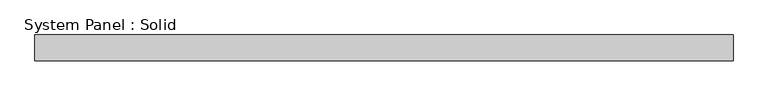
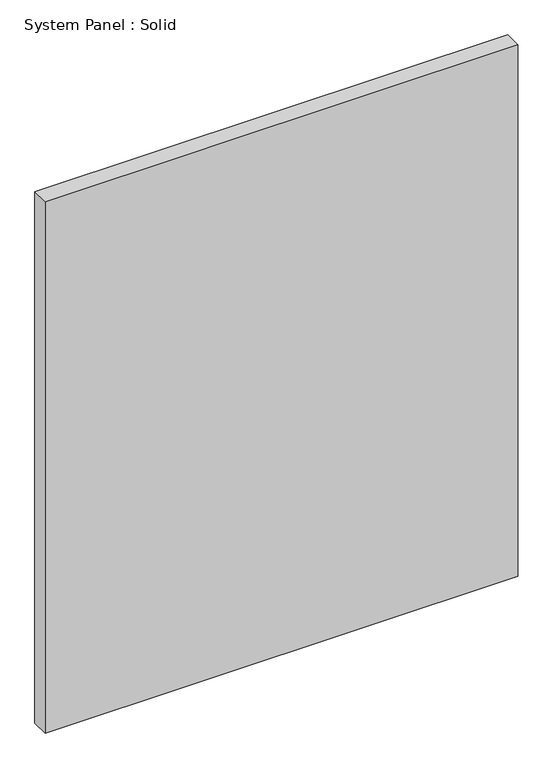
"""IFC4 building model written with IfcOpenShell, lengths in millimetres: plate geometry, System Panel : Solid."""

from ifc_helpers import new_model, si_unit, origin, origin_with_axes, place, context, project, spatial, polyline, outline, extrude, source, transform, mapped, element, save


def system_panel_solid_ede99fb6(model_context):
    return source(origin(), model_context, "Body", "SweptSolid", [
        extrude(outline(polyline([(810.0, -10.5), (-810.0, -10.5), (-810.0, 49.5), (810.0, 49.5), (810.0, -10.5)])), origin_with_axes(), (0.0, 0.0, 1.0), 1925.0),
    ])


if __name__ == "__main__":
    model = new_model("IFC4")
    model_context = context("Model", 3, world=origin())
    ifc_project = project(units=[si_unit("LENGTHUNIT", "METRE", prefix="MILLI")], contexts=[model_context])
    site = spatial("IfcSite", under=ifc_project)
    building = spatial("IfcBuilding", under=site)
    placement = place(None, origin())
    system_panel_solid_shape = system_panel_solid_ede99fb6(model_context)
    element("IfcPlate", 1, ObjectType="System Panel : Solid", at=placement, inside=building, context=model_context, shape_type="MappedRepresentation", body=[
        mapped(system_panel_solid_shape, transform((0.0, 0.0, 0.0), x_axis=(1.0, 0.0, 0.0), y_axis=(0.0, 1.0, 0.0), z_axis=(0.0, 0.0, 1.0))),
    ])
    save(model, "model.ifc")

# Revit data of these elements
# Element 1 (IfcPlate, "System Panel : Solid")
#   Materials on its faces: "Default"
# Materials
#   "Default": class "Miscellaneous", colour RGB 127 127 127, transparency 0
